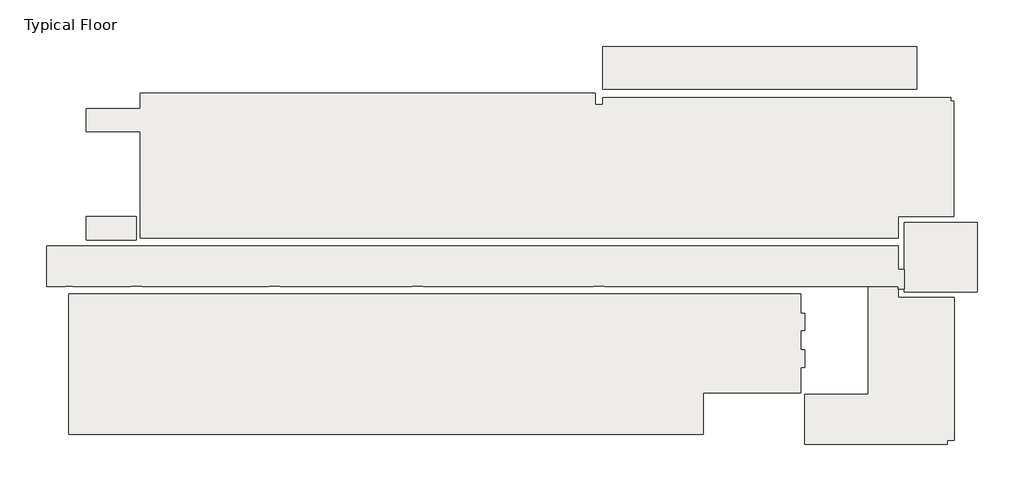
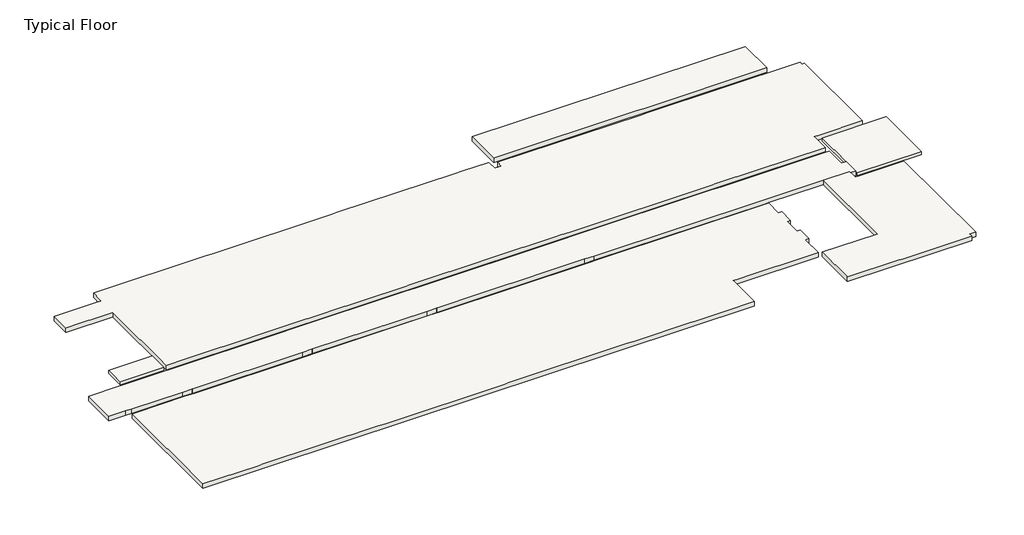
# One storey: 7 slabs.
"""IFC4 building model written with IfcOpenShell, lengths in millimetres."""

from ifc_helpers import new_model, si_unit, frame, origin, place, context, project, spatial, polyline, outline, extrude, faceted_brep, element, save

model = new_model("IFC4")

# Units and contexts
model_context = context("Model", 3, world=origin())
ifc_project = project(units=[si_unit("LENGTHUNIT", "METRE", prefix="MILLI")], contexts=[model_context])

# Site, building, storey
site = spatial("IfcSite", under=ifc_project)
building = spatial("IfcBuilding", under=site)
storey = spatial("IfcBuildingStorey", under=building, Name="Typical Floor", Elevation=3800.0)

# Slabs
placement = place(None, origin())
element("IfcSlab", 1, ObjectType="20", at=placement, inside=storey, context=model_context, shape_type="Brep", body=[
    faceted_brep([(29339.6053211, 1458.6282173, 3600.0), (29339.6053211, -2141.3717827, 3600.0), (25540.6606912, -2141.3717827, 3600.0), (25540.6606912, -992.8836023, 3600.0), (25541.4195047, -992.8836023, 3600.0), (25541.4195047, 1458.6282173, 3600.0), (29339.6053211, -2141.3717827, 3800.0), (29339.6053211, 1458.6282173, 3800.0), (25541.4195047, 1458.6282173, 3800.0), (25541.4195047, -992.8836023, 3800.0), (25540.6606912, -992.8836023, 3800.0), (25540.6606912, -1996.3717827, 3800.0), (25540.6606912, -2141.3717827, 3800.0)], [[[0, 1, 2, 3, 4, 5]], [[6, 7, 8, 9, 10, 11, 12]], [[1, 0, 7, 6]], [[2, 1, 6, 12]], [[2, 12, 11, 10, 3]], [[7, 0, 5, 8]], [[4, 9, 8, 5]], [[9, 4, 3, 10]]]),
])
element("IfcSlab", 2, ObjectType="20", at=placement, inside=storey, context=model_context, shape_type="SweptSolid", body=[
    extrude(outline(polyline([(-14212.0714244, 1758.6282173), (-14212.0714244, 545.3255739), (-16809.1027603, 545.3255739), (-16809.1027603, 1758.6282173), (-14212.0714244, 1758.6282173)])), frame((0.0, 0.0, 3600.0), z_axis=(0.0, 0.0, 1.0), x_axis=(1.0, 0.0, 0.0)), (0.0, 0.0, 1.0), 200.0),
])
element("IfcSlab", 3, ObjectType="28", at=placement, inside=storey, context=model_context, shape_type="Brep", body=[
    faceted_brep([(26203.2216506, 8355.3792217, 3520.0), (9943.2216506, 8355.3792217, 3520.0), (9943.2216506, 10575.3792217, 3520.0), (26203.2216506, 10575.3792217, 3520.0), (26203.2216506, 8355.3792217, 3800.0), (26203.2216506, 10575.3792217, 3800.0), (9943.2216506, 10575.3792217, 3800.0), (9943.2216506, 8551.6453791, 3800.0), (9943.2216506, 8355.3792217, 3800.0), (18471.5975134, 8355.3792217, 3800.0), (18871.5975134, 8355.3792217, 3800.0)], [[[0, 1, 2, 3]], [[4, 5, 6, 7, 8, 9, 10]], [[1, 0, 4, 10, 9, 8]], [[2, 1, 8, 7, 6]], [[3, 2, 6, 5]], [[0, 3, 5, 4]]]),
])
element("IfcSlab", 4, ObjectType="28", at=placement, inside=storey, context=model_context, shape_type="Brep", body=[
    faceted_brep([(28101.2236194, 7751.6453791, 3520.0), (28101.2236194, 1758.6282173, 3520.0), (25541.4195047, 1758.6282173, 3520.0), (25241.4195047, 1758.6282173, 3520.0), (25241.4195047, 645.3255739, 3520.0), (-14012.0714244, 645.3255739, 3520.0), (-14012.0714244, 5957.8562202, 3520.0), (-14012.0714244, 6157.8562202, 3520.0), (-16809.1027603, 6157.8562202, 3520.0), (-16809.1027603, 7355.2095413, 3520.0), (-16709.1027603, 7355.2095413, 3520.0), (-14307.5920656, 7355.2095413, 3520.0), (-14007.5920656, 7355.2095413, 3520.0), (-14007.5920656, 7555.2095413, 3520.0), (-14007.5920656, 8151.3324092, 3520.0), (9543.2216506, 8151.3324092, 3520.0), (9543.2216506, 7551.6453791, 3520.0), (9943.2216506, 7551.6453791, 3520.0), (9943.2216506, 7925.3792217, 3520.0), (18471.5975134, 7925.3792217, 3520.0), (18871.5975134, 7925.3792217, 3520.0), (27951.2236194, 7925.3792217, 3520.0), (27951.2236194, 7751.6453791, 3520.0), (28101.2236194, 1758.6282173, 3800.0), (28101.2236194, 7751.6453791, 3800.0), (27951.2236194, 7751.6453791, 3800.0), (27951.2236194, 7925.3792217, 3800.0), (18871.5975134, 7925.3792217, 3800.0), (18471.5975134, 7925.3792217, 3800.0), (9943.2216506, 7925.3792217, 3800.0), (9943.2216506, 7551.6453791, 3800.0), (9543.2216506, 7551.6453791, 3800.0), (9543.2216506, 8151.3324092, 3800.0), (7948.8072182, 8151.3324092, 3800.0), (7548.8072182, 8151.3324092, 3800.0), (551.39348, 8151.3324092, 3800.0), (151.39348, 8151.3324092, 3800.0), (-6857.9830653, 8151.3324092, 3800.0), (-7257.9830653, 8151.3324092, 3800.0), (-14007.5920656, 8151.3324092, 3800.0), (-14007.5920656, 7555.2095413, 3800.0), (-14007.5920656, 7355.2095413, 3800.0), (-14307.5920656, 7355.2095413, 3800.0), (-16709.1027603, 7355.2095413, 3800.0), (-16809.1027603, 7355.2095413, 3800.0), (-16809.1027603, 6157.8562202, 3800.0), (-14012.0714244, 6157.8562202, 3800.0), (-14012.0714244, 5957.8562202, 3800.0), (-14012.0714244, 645.3255739, 3800.0), (-7357.9791944, 645.3255739, 3800.0), (-6757.9791944, 645.3255739, 3800.0), (51.396575, 645.3255739, 3800.0), (651.396575, 645.3255739, 3800.0), (9443.2258738, 645.3255739, 3800.0), (10043.2258738, 645.3255739, 3800.0), (18292.1885308, 645.3255739, 3800.0), (18892.1885308, 645.3255739, 3800.0), (25241.4195047, 645.3255739, 3800.0), (25241.4195047, 1758.6282173, 3800.0), (25541.4195047, 1758.6282173, 3800.0)], [[[0, 1, 2, 3, 4, 5, 6, 7, 8, 9, 10, 11, 12, 13, 14, 15, 16, 17, 18, 19, 20, 21, 22]], [[23, 24, 25, 26, 27, 28, 29, 30, 31, 32, 33, 34, 35, 36, 37, 38, 39, 40, 41, 42, 43, 44, 45, 46, 47, 48, 49, 50, 51, 52, 53, 54, 55, 56, 57, 58, 59]], [[1, 0, 24, 23]], [[1, 23, 59, 58, 3, 2]], [[4, 3, 58, 57]], [[5, 4, 57, 56, 55, 54, 53, 52, 51, 50, 49, 48]], [[5, 48, 47, 46, 7, 6]], [[8, 7, 46, 45]], [[9, 8, 45, 44]], [[9, 44, 43, 42, 41, 12, 11, 10]], [[12, 41, 40, 39, 14, 13]], [[15, 14, 39, 38, 37, 36, 35, 34, 33, 32]], [[16, 15, 32, 31]], [[17, 16, 31, 30]], [[18, 17, 30, 29]], [[18, 29, 28, 27, 26, 21, 20, 19]], [[22, 21, 26, 25]], [[0, 22, 25, 24]]]),
])
element("IfcSlab", 5, ObjectType="28", at=placement, inside=storey, context=model_context, shape_type="Brep", body=[
    faceted_brep([(25241.4195047, 245.3255739, 3520.0), (25241.4195047, -992.8836023, 3520.0), (25540.6606912, -992.8836023, 3520.0), (25540.6606912, -1996.3717827, 3520.0), (25241.4195047, -1996.3717827, 3520.0), (25241.4195047, -1851.1339506, 3520.0), (23696.3370418, -1851.1339506, 3520.0), (23496.3370418, -1851.1339506, 3520.0), (20396.3370418, -1851.1339506, 3520.0), (20196.3370418, -1851.1339506, 3520.0), (10043.2216506, -1851.1339506, 3520.0), (10043.2216506, -1849.6811448, 3520.0), (9443.2216506, -1849.6811448, 3520.0), (9443.2216506, -1851.1339506, 3520.0), (651.39348, -1851.1339506, 3520.0), (651.39348, -1849.6811448, 3520.0), (51.39348, -1849.6811448, 3520.0), (51.39348, -1851.1339506, 3520.0), (-6757.9830653, -1851.1339506, 3520.0), (-6757.9830653, -1849.6811448, 3520.0), (-7357.9830653, -1849.6811448, 3520.0), (-7357.9830653, -1851.1339506, 3520.0), (-13909.6091474, -1851.1339506, 3520.0), (-13909.6091474, -1849.6811448, 3520.0), (-14509.6091474, -1849.6811448, 3520.0), (-14509.6091474, -1851.1339506, 3520.0), (-17507.5957255, -1851.1339506, 3520.0), (-17507.5957255, -1849.6811448, 3520.0), (-17907.5957255, -1849.6811448, 3520.0), (-17907.5957255, -1851.1339506, 3520.0), (-18867.5920656, -1851.1339506, 3520.0), (-18867.5920656, -1849.6811448, 3520.0), (-18867.5920656, 245.3255739, 3520.0), (25241.4195047, -992.8836023, 3800.0), (25241.4195047, 245.3255739, 3800.0), (18892.1885308, 245.3255739, 3800.0), (18292.1885308, 245.3255739, 3800.0), (10043.2258738, 245.3255739, 3800.0), (9443.2258738, 245.3255739, 3800.0), (651.396575, 245.3255739, 3800.0), (51.396575, 245.3255739, 3800.0), (-6757.9791944, 245.3255739, 3800.0), (-7357.9791944, 245.3255739, 3800.0), (-14012.0714244, 245.3255739, 3800.0), (-14212.0714244, 245.3255739, 3800.0), (-16809.1027603, 245.3255739, 3800.0), (-17009.1027603, 245.3255739, 3800.0), (-18867.5920656, 245.3255739, 3800.0), (-18867.5920656, -1849.6811448, 3800.0), (-18867.5920656, -1851.1339506, 3800.0), (-17907.5957255, -1851.1339506, 3800.0), (-17907.5957255, -1849.6811448, 3800.0), (-17507.5957255, -1849.6811448, 3800.0), (-17507.5957255, -1851.1339506, 3800.0), (-14509.6091474, -1851.1339506, 3800.0), (-14509.6091474, -1849.6811448, 3800.0), (-13909.6091474, -1849.6811448, 3800.0), (-13909.6091474, -1851.1339506, 3800.0), (-7357.9830653, -1851.1339506, 3800.0), (-7357.9830653, -1849.6811448, 3800.0), (-6757.9830653, -1849.6811448, 3800.0), (-6757.9830653, -1851.1339506, 3800.0), (51.39348, -1851.1339506, 3800.0), (51.39348, -1849.6811448, 3800.0), (651.39348, -1849.6811448, 3800.0), (651.39348, -1851.1339506, 3800.0), (9443.2216506, -1851.1339506, 3800.0), (9443.2216506, -1849.6811448, 3800.0), (10043.2216506, -1849.6811448, 3800.0), (10043.2216506, -1851.1339506, 3800.0), (20196.3370418, -1851.1339506, 3800.0), (23496.3370418, -1851.1339506, 3800.0), (23696.3370418, -1851.1339506, 3800.0), (25241.4195047, -1851.1339506, 3800.0), (25241.4195047, -1996.3717827, 3800.0), (25540.6606912, -1996.3717827, 3800.0), (25540.6606912, -992.8836023, 3800.0), (25540.6606912, -992.8836023, 3600.0)], [[[0, 1, 2, 3, 4, 5, 6, 7, 8, 9, 10, 11, 12, 13, 14, 15, 16, 17, 18, 19, 20, 21, 22, 23, 24, 25, 26, 27, 28, 29, 30, 31, 32]], [[33, 34, 35, 36, 37, 38, 39, 40, 41, 42, 43, 44, 45, 46, 47, 48, 49, 50, 51, 52, 53, 54, 55, 56, 57, 58, 59, 60, 61, 62, 63, 64, 65, 66, 67, 68, 69, 70, 71, 72, 73, 74, 75, 76]], [[1, 0, 34, 33]], [[2, 1, 33, 76, 77]], [[3, 2, 77, 76, 75]], [[4, 3, 75, 74]], [[5, 4, 74, 73]], [[49, 30, 29, 50]], [[53, 26, 25, 54]], [[57, 22, 21, 58]], [[61, 18, 17, 62]], [[13, 66, 65, 14]], [[5, 73, 72, 71, 70, 69, 10, 9, 8, 7, 6]], [[32, 31, 30, 49, 48, 47]], [[0, 32, 47, 46, 45, 44, 43, 42, 41, 40, 39, 38, 37, 36, 35, 34]], [[52, 27, 26, 53]], [[28, 51, 50, 29]], [[51, 28, 27, 52]], [[23, 56, 55, 24]], [[56, 23, 22, 57]], [[24, 55, 54, 25]], [[19, 60, 59, 20]], [[60, 19, 18, 61]], [[20, 59, 58, 21]], [[11, 68, 67, 12]], [[68, 11, 10, 69]], [[12, 67, 66, 13]], [[15, 64, 63, 16]], [[64, 15, 14, 65]], [[16, 63, 62, 17]]]),
])
element("IfcSlab", 6, ObjectType="28", at=placement, inside=storey, context=model_context, shape_type="Brep", body=[
    faceted_brep([(28136.856558, -2441.3717827, 3520.0), (28136.856558, -9844.9662281, 3520.0), (27784.8345171, -9844.9662281, 3520.0), (27784.8345171, -10044.9662281, 3520.0), (20395.2300261, -10044.9662281, 3520.0), (20395.2300261, -7451.1339506, 3520.0), (23696.3370418, -7451.1339506, 3520.0), (23696.3370418, -7251.1339506, 3520.0), (23696.3370418, -1851.1339506, 3520.0), (25241.4195047, -1851.1339506, 3520.0), (25241.4195047, -1996.3717827, 3520.0), (25240.6606912, -1996.3717827, 3520.0), (25240.6606912, -2441.3717827, 3520.0), (28136.856558, -9844.9662281, 3800.0), (28136.856558, -2441.3717827, 3800.0), (25540.6606912, -2441.3717827, 3800.0), (25240.6606912, -2441.3717827, 3800.0), (25240.6606912, -1996.3717827, 3800.0), (25241.4195047, -1996.3717827, 3800.0), (25241.4195047, -1851.1339506, 3800.0), (23696.3370418, -1851.1339506, 3800.0), (23696.3370418, -7251.1339506, 3800.0), (23696.3370418, -7451.1339506, 3800.0), (20395.2300261, -7451.1339506, 3800.0), (20395.2300261, -7571.4322554, 3800.0), (20395.2300261, -7584.1322554, 3800.0), (20395.2300261, -9947.194205, 3800.0), (20395.2300261, -10044.9662281, 3800.0), (23445.2926489, -10044.9662281, 3800.0), (23695.2926489, -10044.9662281, 3800.0), (27784.8345171, -10044.9662281, 3800.0), (27784.8345171, -9844.9662281, 3800.0)], [[[0, 1, 2, 3, 4, 5, 6, 7, 8, 9, 10, 11, 12]], [[13, 14, 15, 16, 17, 18, 19, 20, 21, 22, 23, 24, 25, 26, 27, 28, 29, 30, 31]], [[9, 19, 18, 10]], [[14, 0, 12, 16, 15]], [[1, 0, 14, 13]], [[2, 1, 13, 31]], [[3, 2, 31, 30]], [[4, 3, 30, 29, 28, 27]], [[5, 4, 27, 26, 25, 24, 23]], [[6, 5, 23, 22]], [[6, 22, 21, 20, 8, 7]], [[9, 8, 20, 19]], [[11, 17, 16, 12]], [[17, 11, 10, 18]]]),
])
element("IfcSlab", 7, ObjectType="28", at=placement, inside=storey, context=model_context, shape_type="Brep", body=[
    faceted_brep([(20196.3370418, -2249.6811448, 3520.0), (20196.3370418, -3251.1339506, 3520.0), (20396.3370418, -3251.1339506, 3520.0), (20396.3370418, -4150.7725523, 3520.0), (20196.3370418, -4150.7725523, 3520.0), (20196.3370418, -5149.7829976, 3520.0), (20396.3370418, -5149.7829976, 3520.0), (20396.3370418, -6051.4322554, 3520.0), (20395.2300261, -6051.4322554, 3520.0), (20195.2300261, -6051.4322554, 3520.0), (20195.2300261, -7371.4322554, 3520.0), (15344.7363769, -7371.4322554, 3520.0), (15144.7363769, -7371.4322554, 3520.0), (15144.7363769, -7771.4322554, 3520.0), (15144.7363769, -9540.2012066, 3520.0), (-17707.5957255, -9540.2012066, 3520.0), (-17707.5957255, -2249.6811448, 3520.0), (20196.3370418, -3251.1339506, 3800.0), (20196.3370418, -2249.6811448, 3800.0), (10043.2216506, -2249.6811448, 3800.0), (9443.2216506, -2249.6811448, 3800.0), (651.39348, -2249.6811448, 3800.0), (51.39348, -2249.6811448, 3800.0), (-6757.9830653, -2249.6811448, 3800.0), (-7357.9830653, -2249.6811448, 3800.0), (-13909.6091474, -2249.6811448, 3800.0), (-14509.6091474, -2249.6811448, 3800.0), (-17507.5957255, -2249.6811448, 3800.0), (-17707.5957255, -2249.6811448, 3800.0), (-17707.5957255, -9540.2012066, 3800.0), (-14512.2396142, -9540.2012066, 3800.0), (-14112.2396142, -9540.2012066, 3800.0), (-7257.9830653, -9540.2012066, 3800.0), (-6857.9830653, -9540.2012066, 3800.0), (151.39348, -9540.2012066, 3800.0), (551.39348, -9540.2012066, 3800.0), (7548.8072182, -9540.2012066, 3800.0), (7948.8072182, -9540.2012066, 3800.0), (14942.1345122, -9540.2012066, 3800.0), (15144.7363769, -9540.2012066, 3800.0), (15144.7363769, -7771.4322554, 3800.0), (15144.7363769, -7371.4322554, 3800.0), (15344.7363769, -7371.4322554, 3800.0), (20195.2300261, -7371.4322554, 3800.0), (20195.2300261, -6051.4322554, 3800.0), (20395.2300261, -6051.4322554, 3800.0), (20396.3370418, -6051.4322554, 3800.0), (20396.3370418, -5149.7829976, 3800.0), (20196.3370418, -5149.7829976, 3800.0), (20196.3370418, -4150.7725523, 3800.0), (20396.3370418, -4150.7725523, 3800.0), (20396.3370418, -3251.1339506, 3800.0)], [[[0, 1, 2, 3, 4, 5, 6, 7, 8, 9, 10, 11, 12, 13, 14, 15, 16]], [[17, 18, 19, 20, 21, 22, 23, 24, 25, 26, 27, 28, 29, 30, 31, 32, 33, 34, 35, 36, 37, 38, 39, 40, 41, 42, 43, 44, 45, 46, 47, 48, 49, 50, 51]], [[1, 0, 18, 17]], [[2, 1, 17, 51]], [[3, 2, 51, 50]], [[4, 3, 50, 49]], [[5, 4, 49, 48]], [[6, 5, 48, 47]], [[7, 6, 47, 46]], [[7, 46, 45, 44, 9, 8]], [[10, 9, 44, 43]], [[10, 43, 42, 41, 12, 11]], [[12, 41, 40, 39, 14, 13]], [[15, 14, 39, 38, 37, 36, 35, 34, 33, 32, 31, 30, 29]], [[16, 15, 29, 28]], [[0, 16, 28, 27, 26, 25, 24, 23, 22, 21, 20, 19, 18]]]),
])

save(model, "model.ifc")

# Revit data of these elements
# Type "20"
#   Function = 0
#   Layers, outside or top first: 20 cm "Concrete" (function 1)
# Type "28"
#   Function = 0
#   Layers, outside or top first: 28 cm "Concrete" (function 1)
# Element 1 (IfcSlab, "20")
#   Mark = "S1"
#   SOFiSTiK_AMG_Comments = ""
#   Height Offset From Level = 0 cm
#   built-in parameter 1001954 = 1
#   SOFiSTiK_AMG_Scheduled = yes
#   SOFiSTiK_AMG_Adjusted = yes
#   Phase Created = New Construction
#   Materials on its faces: "Concrete"
# Element 2 (IfcSlab, "20")
#   Mark = "S2"
#   SOFiSTiK_AMG_Comments = ""
#   Height Offset From Level = 0 cm
#   built-in parameter 1001954 = 1
#   SOFiSTiK_AMG_Scheduled = yes
#   SOFiSTiK_AMG_Adjusted = yes
#   Phase Created = New Construction
#   Materials on its faces: "Concrete"
# Element 3 (IfcSlab, "28")
#   Mark = "S3"
#   SOFiSTiK_AMG_Comments = ""
#   Height Offset From Level = 0 cm
#   built-in parameter 1001954 = 1
#   SOFiSTiK_AMG_Scheduled = yes
#   SOFiSTiK_AMG_Adjusted = yes
#   Phase Created = New Construction
#   Materials on its faces: "Concrete"
# Element 4 (IfcSlab, "28")
#   Mark = "S4"
#   SOFiSTiK_AMG_Comments = ""
#   Height Offset From Level = 0 cm
#   built-in parameter 1001954 = 1
#   SOFiSTiK_AMG_Scheduled = yes
#   SOFiSTiK_AMG_Adjusted = no
#   Phase Created = New Construction
#   Materials on its faces: "Concrete"
# Element 5 (IfcSlab, "28")
#   Mark = "S5"
#   SOFiSTiK_AMG_Comments = ""
#   Height Offset From Level = 0 cm
#   built-in parameter 1001954 = 1
#   SOFiSTiK_AMG_Scheduled = yes
#   SOFiSTiK_AMG_Adjusted = yes
#   Phase Created = New Construction
#   Materials on its faces: "Concrete"
# Element 6 (IfcSlab, "28")
#   Mark = "S6"
#   SOFiSTiK_AMG_Comments = ""
#   Height Offset From Level = 0 cm
#   built-in parameter 1001954 = 1
#   SOFiSTiK_AMG_Scheduled = yes
#   SOFiSTiK_AMG_Adjusted = yes
#   Phase Created = New Construction
#   Materials on its faces: "Concrete"
# Element 7 (IfcSlab, "28")
#   Mark = "S7"
#   SOFiSTiK_AMG_Comments = ""
#   Height Offset From Level = 0 cm
#   built-in parameter 1001954 = 1
#   SOFiSTiK_AMG_Scheduled = yes
#   SOFiSTiK_AMG_Adjusted = yes
#   Phase Created = New Construction
#   Materials on its faces: "Concrete"
# Materials
#   "Concrete": class "Concrete", colour RGB 192 192 192, transparency 0, Keynote = "01000", Description = "Cast-in-place concrete", Cost = 0
